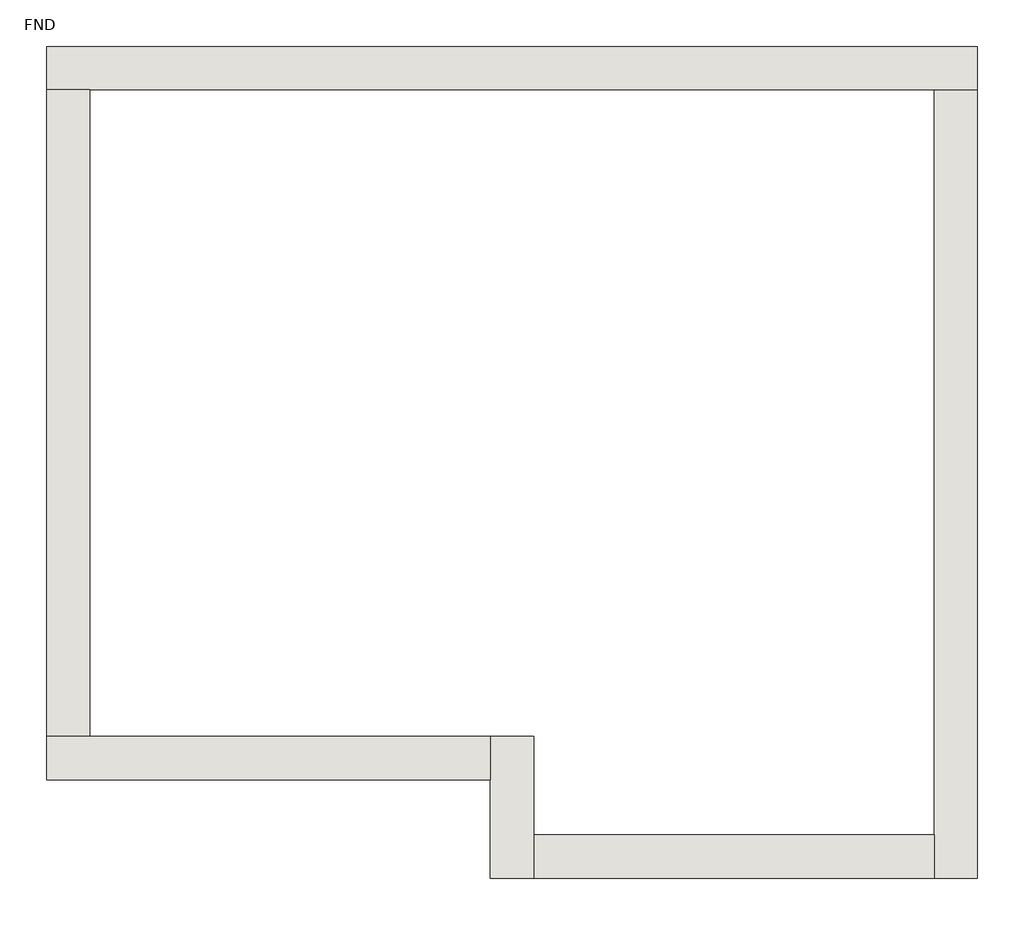
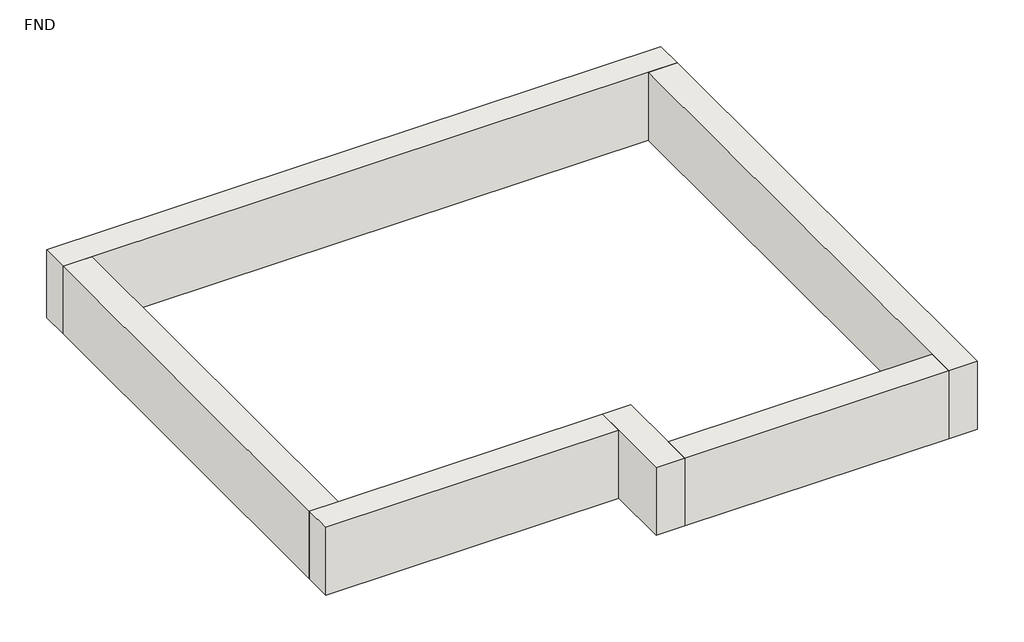
# One storey: 6 walls.
"""IFC4 building model written with IfcOpenShell, lengths in millimetres."""

from ifc_helpers import new_model, si_unit, frame, origin, place, context, project, spatial, polyline, outline, extrude, faceted_brep, element, save

model = new_model("IFC4")

# Units and contexts
model_context = context("Model", 3, world=origin())
ifc_project = project(units=[si_unit("LENGTHUNIT", "METRE", prefix="MILLI")], contexts=[model_context])

# Site, building, storey
site = spatial("IfcSite", under=ifc_project)
building = spatial("IfcBuilding", under=site)
storey = spatial("IfcBuildingStorey", under=building, Name="FND", Elevation=-1100.0)

# Walls
placement = place(None, origin())
element("IfcWall", 1, ObjectType="Wall-Fnd_440Blk", at=placement, inside=storey, context=model_context, shape_type="Brep", body=[
    faceted_brep([(-8592.9479488, 3921.8593841, -1100.0), (-8152.9479488, 3921.8593841, -1100.0), (407.0520512, 3921.8593841, -1100.0), (847.0520512, 3921.8593841, -1100.0), (847.0520512, 3921.8593841, 0.0), (407.0520512, 3921.8593841, 0.0), (-8152.9479488, 3921.8593841, 0.0), (-8592.9479488, 3921.8593841, 0.0), (-8592.9479488, 4361.8593841, -1100.0), (-8592.9479488, 4361.8593841, 0.0), (847.0520512, 4361.8593841, 0.0), (847.0520512, 4361.8593841, -1100.0)], [[[0, 1, 2, 3, 4, 5, 6, 7]], [[8, 9, 10, 11]], [[3, 2, 1, 0, 8, 11]], [[7, 6, 5, 4, 10, 9]], [[4, 3, 11, 10]], [[0, 7, 9, 8]]]),
])
element("IfcWall", 2, ObjectType="Wall-Fnd_440Blk", at=placement, inside=storey, context=model_context, shape_type="Brep", body=[
    faceted_brep([(407.0520512, 3921.8593841, -1100.0), (407.0520512, -3638.1406159, -1100.0), (407.0520512, -4078.1406159, -1100.0), (407.0520512, -4078.1406159, 0.0), (407.0520512, -3638.1406159, 0.0), (407.0520512, 3921.8593841, 0.0), (847.0520512, 3921.8593841, -1100.0), (847.0520512, 3921.8593841, 0.0), (847.0520512, -4078.1406159, 0.0), (847.0520512, -4078.1406159, -1100.0)], [[[0, 1, 2, 3, 4, 5]], [[6, 7, 8, 9]], [[2, 1, 0, 6, 9]], [[5, 4, 3, 8, 7]], [[0, 5, 7, 6]], [[3, 2, 9, 8]]]),
])
element("IfcWall", 3, ObjectType="Wall-Fnd_440Blk", at=placement, inside=storey, context=model_context, shape_type="SweptSolid", body=[
    extrude(outline(polyline([(-3652.9479488, -3638.1406159), (407.0520512, -3638.1406159), (407.0520512, -4078.1406159), (-3652.9479488, -4078.1406159), (-3652.9479488, -3638.1406159)])), frame((0.0, 0.0, -1100.0), z_axis=(0.0, 0.0, 1.0), x_axis=(1.0, 0.0, 0.0)), (0.0, 0.0, 1.0), 1100.0),
])
element("IfcWall", 4, ObjectType="Wall-Fnd_440Blk", at=placement, inside=storey, context=model_context, shape_type="Brep", body=[
    faceted_brep([(-3652.9479488, -4078.1406159, -1100.0), (-3652.9479488, -3638.1406159, -1100.0), (-3652.9479488, -2638.1406159, -1100.0), (-3652.9479488, -2638.1406159, 0.0), (-3652.9479488, -3638.1406159, 0.0), (-3652.9479488, -4078.1406159, 0.0), (-4092.9479488, -4078.1406159, -1100.0), (-4092.9479488, -4078.1406159, 0.0), (-4092.9479488, -3078.1406159, 0.0), (-4092.9479488, -2638.1406159, 0.0), (-4092.9479488, -2638.1406159, -1100.0), (-4092.9479488, -3078.1406159, -1100.0)], [[[0, 1, 2, 3, 4, 5]], [[6, 7, 8, 9, 10, 11]], [[2, 1, 0, 6, 11, 10]], [[5, 4, 3, 9, 8, 7]], [[0, 5, 7, 6]], [[3, 2, 10, 9]]]),
])
element("IfcWall", 5, ObjectType="Wall-Fnd_440Blk", at=placement, inside=storey, context=model_context, shape_type="Brep", body=[
    faceted_brep([(-4092.9479488, -2638.1406159, -1100.0), (-8152.9479488, -2638.1406159, -1100.0), (-8592.9479488, -2638.1406159, -1100.0), (-8592.9479488, -2638.1406159, 0.0), (-8152.9479488, -2638.1406159, 0.0), (-4092.9479488, -2638.1406159, 0.0), (-4092.9479488, -3078.1406159, -1100.0), (-4092.9479488, -3078.1406159, 0.0), (-8592.9479488, -3078.1406159, 0.0), (-8592.9479488, -3078.1406159, -1100.0)], [[[0, 1, 2, 3, 4, 5]], [[6, 7, 8, 9]], [[2, 1, 0, 6, 9]], [[5, 4, 3, 8, 7]], [[0, 5, 7, 6]], [[3, 2, 9, 8]]]),
])
element("IfcWall", 6, ObjectType="Wall-Fnd_440Blk", at=placement, inside=storey, context=model_context, shape_type="SweptSolid", body=[
    extrude(outline(polyline([(-8152.9479488, 3921.8593841), (-8152.9479488, -2638.1406159), (-8592.9479488, -2638.1406159), (-8592.9479488, 3921.8593841), (-8152.9479488, 3921.8593841)])), frame((0.0, 0.0, -1100.0), z_axis=(0.0, 0.0, 1.0), x_axis=(1.0, 0.0, 0.0)), (0.0, 0.0, 1.0), 1100.0),
])

save(model, "model.ifc")

# Revit data of these elements
# Project information
#   Project Issue Date = "Issue Date"
#   Project Status = "Project Status"
#   Client Name = "Owner"
#   Project Address = "Enter address here"
#   Project Name = "Project Management Assignment 1"
#   Project Number = "Project Number"
# Type "Wall-Fnd_440Blk"
#   Keynote = "F10"
#   Width = 440 mm
#   Layers, outside or top first: 440 mm "Concrete Masonry Units" (function 1)
# Elements 1, 2, 3, 4, 5, 6 (IfcWall, "Wall-Fnd_440Blk")
#   Top Offset = 0 mm
#   Base Offset = 0 mm
#   wall height = 1100 mm
#   Phase Created = New Construction
#   Base Constraint = FND
#   Top Constraint = 00 Ground
#   Materials on its faces: "Concrete Masonry Units"
# Materials
#   "Concrete Masonry Units": class "Masonry", colour RGB 181 181 181, transparency 0, Description = "Concrete masonry units", Cost = 0
